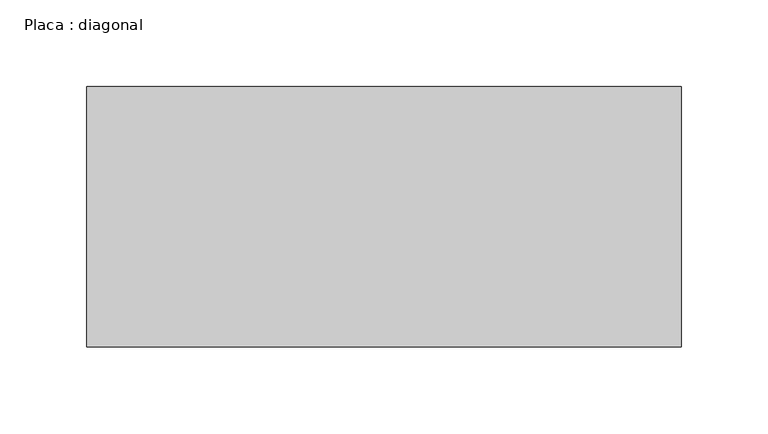
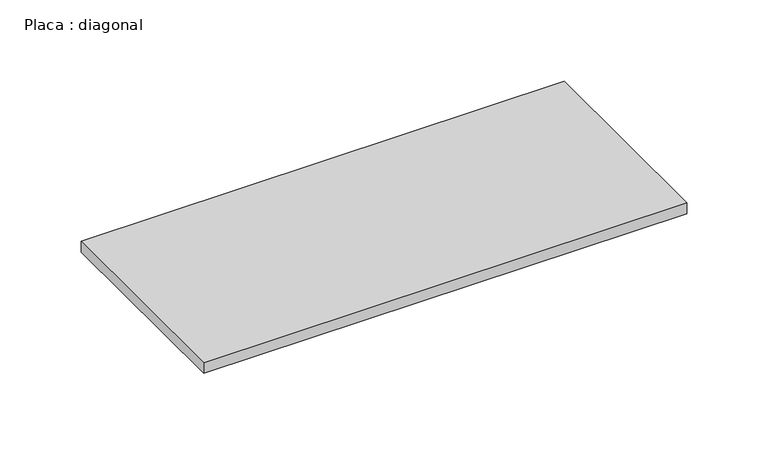
"""IFC4 building model written with IfcOpenShell, lengths in millimetres: beam geometry, Placa : diagonal."""

from ifc_helpers import new_model, si_unit, frame, origin, place, context, project, spatial, polyline, outline, extrude, source, transform, mapped, element, save


def placa_diagonal_acf5f4f6(model_context):
    return source(origin(), model_context, "Body", "SweptSolid", [
        extrude(outline(polyline([(171.6122387, 75.0), (171.6122387, -75.0), (-170.6977756, -75.0), (-170.6977756, 75.0), (171.6122387, 75.0)])), frame((0.0, 0.0, -4.0), z_axis=(0.0, 0.0, 1.0), x_axis=(1.0, 0.0, 0.0)), (0.0, 0.0, 1.0), 8.0),
    ])


if __name__ == "__main__":
    model = new_model("IFC4")
    model_context = context("Model", 3, world=origin())
    ifc_project = project(units=[si_unit("LENGTHUNIT", "METRE", prefix="MILLI")], contexts=[model_context])
    site = spatial("IfcSite", under=ifc_project)
    building = spatial("IfcBuilding", under=site)
    placement = place(None, origin())
    placa_diagonal_shape = placa_diagonal_acf5f4f6(model_context)
    element("IfcBeam", 1, ObjectType="Placa : diagonal", at=placement, inside=building, context=model_context, shape_type="MappedRepresentation", body=[
        mapped(placa_diagonal_shape, transform((0.0, 0.0, 0.0), x_axis=(1.0, 0.0, 0.0), y_axis=(0.0, 1.0, 0.0), z_axis=(0.0, 0.0, 1.0))),
    ])
    save(model, "model.ifc")

# Revit data of these elements
# Type "Placa : diagonal"
#   W = 0
#   Length [instance default] = 1.50 m
#   b = 0.15 m
#   d = 0.008 m
#   A = 0 m²
#   Structural Material [instance default] = Aço, 45-345
# Element 1 (IfcBeam, "Placa : diagonal")
#   Materials on its faces: "Aço, 45-345"
# Materials
#   "Aço, 45-345": class "Metal", colour RGB 247 247 247, transparency 0, Description = "Aço 345 MPa", Cost = 0
